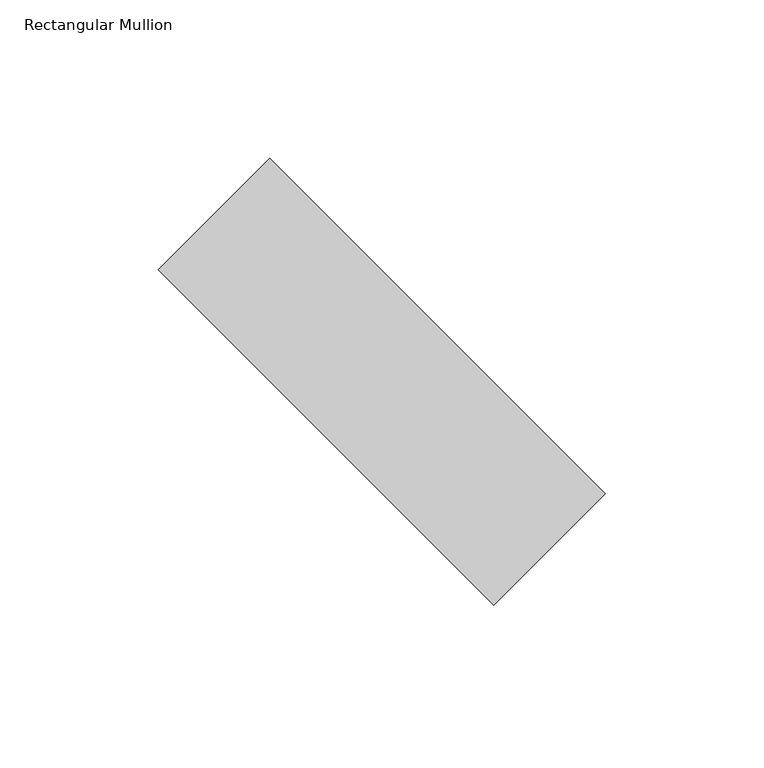
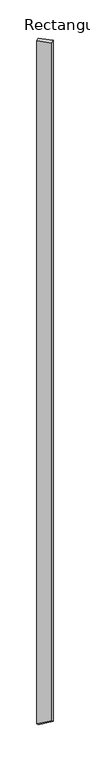
"""IFC4 building model written with IfcOpenShell, lengths in millimetres: member geometry, Rectangular Mullion : tilted mullions."""

import ifcopenshell
import ifcopenshell.guid

model = None  # the IFC model being written
_history = None  # IfcOwnerHistory: only IFC2X3 demands one
_inside = {}  # id of a spatial element -> (the spatial element, [elements in it])
_under = {}  # id of a project, library or spatial element -> (it, [spatial elements below it])
_declared = {}  # id of a project -> (the project, [libraries it declares])
_typed = {}  # id of a type object -> (the type object, [elements of that type])
_made_of = {}  # id of a material, layer set ... -> (it, [elements and type objects made of it])


def new_model(schema):
    """Start an empty IFC model of exactly this schema.

    Asked for "IFC4X3", IfcOpenShell would pick the latest addendum, in which some entities
    have other attributes; the version numbers below select the first issue.
    IFC2X3 requires an IfcOwnerHistory on every rooted entity: one is made here for all.
    """
    global model, _history
    if schema == "IFC4X3":
        model = ifcopenshell.file(schema_version=(4, 3, 0, 0))
    else:
        model = ifcopenshell.file(schema=schema)
    _inside.clear()
    _under.clear()
    _declared.clear()
    _typed.clear()
    _made_of.clear()
    _history = None
    if model.schema == "IFC2X3":
        org = make("IfcOrganization", Name="unknown")
        user = make(
            "IfcPersonAndOrganization",
            ThePerson=make("IfcPerson", FamilyName="unknown"),
            TheOrganization=org,
        )
        app = make(
            "IfcApplication",
            ApplicationDeveloper=org,
            Version="unknown",
            ApplicationFullName="unknown",
            ApplicationIdentifier="unknown",
        )
        _history = make(
            "IfcOwnerHistory",
            OwningUser=user,
            OwningApplication=app,
            ChangeAction="ADDED",
            CreationDate=0,
        )
    return model


def make(cls, **values):
    """One entity of the class cls with the attributes given. An attribute that is None is left unset."""
    return model.create_entity(
        cls, **{name: value for name, value in values.items() if value is not None}
    )


def rooted(cls, **values):
    """An entity with a GlobalId (a new one), such as an element, a storey or a relation."""
    return make(cls, GlobalId=ifcopenshell.guid.new(), OwnerHistory=_history, **values)


def si_unit(unit_type, name, prefix=None):
    """IfcSIUnit, for example si_unit("LENGTHUNIT", "METRE", prefix="MILLI")."""
    return make("IfcSIUnit", UnitType=unit_type, Prefix=prefix, Name=name)


def assignment(units):
    """IfcUnitAssignment: the units of a project."""
    return None if units is None else make("IfcUnitAssignment", Units=units)


def point(xyz):
    """IfcCartesianPoint."""
    return None if xyz is None else make("IfcCartesianPoint", Coordinates=xyz)


def direction(xyz):
    """IfcDirection."""
    return None if xyz is None else make("IfcDirection", DirectionRatios=xyz)


def frame(location, z_axis=None, x_axis=None):
    """IfcAxis2Placement3D, a coordinate frame: its origin and axes. An axis left out is left unset."""
    return make(
        "IfcAxis2Placement3D",
        Location=point(location),
        Axis=direction(z_axis),
        RefDirection=direction(x_axis),
    )


def origin():
    """The frame at (0, 0, 0) with its axes left unset."""
    return frame((0.0, 0.0, 0.0))


def place(relative_to, where):
    """IfcLocalPlacement: puts the frame where relative to a parent placement (None: the world)."""
    return make(
        "IfcLocalPlacement", PlacementRelTo=relative_to, RelativePlacement=where
    )


def context(
    kind, dimensions, precision=None, world=None, true_north=None, identifier=None
):
    """IfcGeometricRepresentationContext, for example the 3D "Model" context."""
    return make(
        "IfcGeometricRepresentationContext",
        ContextIdentifier=identifier,
        ContextType=kind,
        CoordinateSpaceDimension=dimensions,
        Precision=precision,
        WorldCoordinateSystem=world,
        TrueNorth=true_north,
    )


def project(units=None, contexts=None):
    """IfcProject with its units and contexts."""
    return rooted(
        "IfcProject",
        Name="project",
        RepresentationContexts=contexts,
        UnitsInContext=assignment(units),
    )


def spatial(cls, under=None, at=None, **own):
    """A site, building, storey or space (cls), placed at a placement, below another one or the project."""
    s = rooted(cls, ObjectPlacement=at, **own)
    if under is not None:
        _under.setdefault(under.id(), (under, []))[1].append(s)
    return s


def faces_of(points, faces, orient=None, outer=None):
    """IfcFace entities. A face is a list of loops; a loop is a list of indices into points, from 0.

    orient and outer hold one flag for each loop. By default every Orientation is true, the
    first loop of a face is its IfcFaceOuterBound and the others are IfcFaceBound.
    """
    made = []
    for i, loops in enumerate(faces):
        bounds = []
        for j, loop in enumerate(loops):
            is_outer = j == 0 if outer is None else outer[i][j]
            bounds.append(
                make(
                    "IfcFaceOuterBound" if is_outer else "IfcFaceBound",
                    Bound=make("IfcPolyLoop", Polygon=[points[k] for k in loop]),
                    Orientation=True if orient is None else orient[i][j],
                )
            )
        made.append(make("IfcFace", Bounds=bounds))
    return made


def faceted_brep(points, faces, orient=None, outer=None, voids=None):
    """IfcFacetedBrep: a solid bounded by flat faces; with voids (closed shells), ...WithVoids."""
    shared = [point(p) for p in points]
    hull = make("IfcClosedShell", CfsFaces=faces_of(shared, faces, orient, outer))
    if voids is None:
        return make("IfcFacetedBrep", Outer=hull)
    return make(
        "IfcFacetedBrepWithVoids",
        Outer=hull,
        Voids=[
            make(cls, CfsFaces=faces_of(shared, fs, o, b)) for cls, fs, o, b in voids
        ],
    )


def shape(context_of_items, identifier, shape_type, items):
    """IfcShapeRepresentation: the items that make up one representation, for example the "Body"."""
    return make(
        "IfcShapeRepresentation",
        ContextOfItems=context_of_items,
        RepresentationIdentifier=identifier,
        RepresentationType=shape_type,
        Items=items,
    )


def source(mapping_origin, context_of_items, identifier, shape_type, items):
    """IfcRepresentationMap: a shape defined once, which mapped items show again and again."""
    return make(
        "IfcRepresentationMap",
        MappingOrigin=mapping_origin,
        MappedRepresentation=shape(context_of_items, identifier, shape_type, items),
    )


def transform(
    local_origin,
    x_axis=None,
    y_axis=None,
    z_axis=None,
    scale=None,
    scale2=None,
    scale3=None,
    uniform=True,
):
    """IfcCartesianTransformationOperator3D, or its non-uniform kind. x_axis, y_axis, z_axis: its Axis1, 2, 3."""
    if uniform:
        return make(
            "IfcCartesianTransformationOperator3D",
            Axis1=direction(x_axis),
            Axis2=direction(y_axis),
            LocalOrigin=point(local_origin),
            Scale=scale,
            Axis3=direction(z_axis),
        )
    return make(
        "IfcCartesianTransformationOperator3DnonUniform",
        Axis1=direction(x_axis),
        Axis2=direction(y_axis),
        LocalOrigin=point(local_origin),
        Scale=scale,
        Axis3=direction(z_axis),
        Scale2=scale2,
        Scale3=scale3,
    )


def mapped(mapping_source, mapping_target):
    """IfcMappedItem: shows the shape of a source again, moved by a transform."""
    return make(
        "IfcMappedItem", MappingSource=mapping_source, MappingTarget=mapping_target
    )


def made_of(thing, what):
    """Note that an element or type object is made of a material, layer set ...; save() writes the relation."""
    if what is not None:
        _made_of.setdefault(what.id(), (what, []))[1].append(thing)
    return thing


def element(
    cls,
    number,
    at=None,
    inside=None,
    cuts=None,
    type_object=None,
    material=None,
    context=None,
    identifier="Body",
    shape_type=None,
    held_by="IfcProductDefinitionShape",
    body=None,
    shapes=None,
    **own,
):
    """One element of the class cls, such as IfcWall. Its Tag is "e" and its number.

    at: its placement. inside: the storey or other place that contains it. cuts: it is an
    opening in that element (IfcRelVoidsElement). A single representation is given by context,
    identifier, shape_type and body (its items); several are given by shapes. held_by: the class
    of the entity that holds the representations. save() writes the other relations.
    """
    e = rooted(cls, Tag="e%d" % number, ObjectPlacement=at, **own)
    if body is not None:
        shapes = [shape(context, identifier, shape_type, body)]
    if shapes is not None:
        e.Representation = make(held_by, Representations=shapes)
    if inside is not None:
        _inside.setdefault(inside.id(), (inside, []))[1].append(e)
    if cuts is not None:
        rooted(
            "IfcRelVoidsElement", RelatingBuildingElement=cuts, RelatedOpeningElement=e
        )
    if type_object is not None:
        _typed.setdefault(type_object.id(), (type_object, []))[1].append(e)
    return made_of(e, material)


def aggregate(whole, parts):
    """IfcRelAggregates: a whole, such as a stair, and the parts it consists of."""
    return rooted("IfcRelAggregates", RelatingObject=whole, RelatedObjects=parts)


def save(model, path):
    """Write the relations noted so far, then the file.

    IfcRelAggregates (storeys below a building ...), IfcRelContainedInSpatialStructure (elements
    in a storey), IfcRelDefinesByType, IfcRelAssociatesMaterial and IfcRelDeclares: one each for
    every whole, place, type object, material and project.
    """
    for whole, parts in _under.values():
        aggregate(whole, parts)
    for where, things in _inside.values():
        rooted(
            "IfcRelContainedInSpatialStructure",
            RelatedElements=things,
            RelatingStructure=where,
        )
    for kind, things in _typed.values():
        rooted("IfcRelDefinesByType", RelatedObjects=things, RelatingType=kind)
    for what, things in _made_of.values():
        rooted("IfcRelAssociatesMaterial", RelatedObjects=things, RelatingMaterial=what)
    for by, libraries in _declared.values():
        rooted("IfcRelDeclares", RelatingContext=by, RelatedDefinitions=libraries)
    model.write(path)


def rectangular_mullion_e764de33(model_context):
    return source(origin(), model_context, "Body", "Brep", [
        faceted_brep([(-35.3553391, 70.7106781, 0.0), (-70.7106781, 35.3553391, 0.0), (35.3553391, -70.7106781, 0.0), (70.7106781, -35.3553391, 0.0), (-35.3553391, 70.7106781, -8054.5115791), (-70.7106781, 35.3553391, -8009.4581263), (35.3553391, -70.7106781, -7944.4067811), (70.7106781, -35.3553391, -7989.4602339)], [[[0, 1, 2, 3]], [[1, 0, 4, 5]], [[2, 1, 5, 6]], [[3, 2, 6, 7]], [[0, 3, 7, 4]], [[4, 7, 6, 5]]]),
    ])


if __name__ == "__main__":
    model = new_model("IFC4")
    model_context = context("Model", 3, world=origin())
    ifc_project = project(units=[si_unit("LENGTHUNIT", "METRE", prefix="MILLI")], contexts=[model_context])
    site = spatial("IfcSite", under=ifc_project)
    building = spatial("IfcBuilding", under=site)
    placement = place(None, origin())
    rectangular_mullion_shape = rectangular_mullion_e764de33(model_context)
    element("IfcMember", 1, ObjectType="Rectangular Mullion : tilted mullions", at=placement, inside=building, context=model_context, shape_type="MappedRepresentation", body=[
        mapped(rectangular_mullion_shape, transform((0.0, 0.0, 0.0), x_axis=(1.0, 0.0, 0.0), y_axis=(0.0, 1.0, 0.0), z_axis=(0.0, 0.0, 1.0))),
    ])
    save(model, "model.ifc")

# Revit data of these elements
# Type "Rectangular Mullion : tilted mullions"
#   built-in parameter 1007304 = 0.492126 (stored number, unit not read)
#   built-in parameter 1007301 = 0.082021 (stored number, unit not read)
#   built-in parameter 1007300 = 0.082021 (stored number, unit not read)
# Element 1 (IfcMember, "Rectangular Mullion : tilted mullions")
#   Materials on its faces: "Aluminum"
# Materials
#   "Aluminum": class "Metal", colour RGB 244 244 244, transparency 0, Description = "Aluminum 6061", Cost = 0
